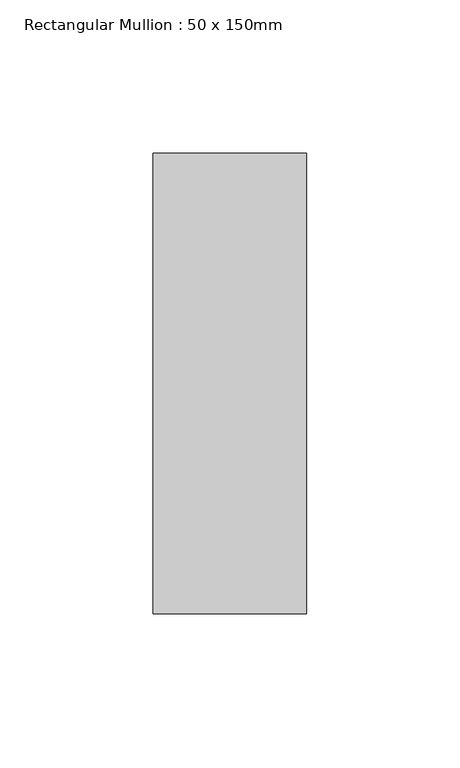
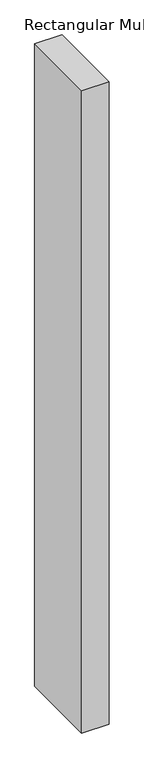
"""IFC4 building model written with IfcOpenShell, lengths in millimetres: member geometry, Rectangular Mullion : 50 x 150mm."""

import ifcopenshell
import ifcopenshell.guid

model = None  # the IFC model being written
_history = None  # IfcOwnerHistory: only IFC2X3 demands one
_inside = {}  # id of a spatial element -> (the spatial element, [elements in it])
_under = {}  # id of a project, library or spatial element -> (it, [spatial elements below it])
_declared = {}  # id of a project -> (the project, [libraries it declares])
_typed = {}  # id of a type object -> (the type object, [elements of that type])
_made_of = {}  # id of a material, layer set ... -> (it, [elements and type objects made of it])


def new_model(schema):
    """Start an empty IFC model of exactly this schema.

    Asked for "IFC4X3", IfcOpenShell would pick the latest addendum, in which some entities
    have other attributes; the version numbers below select the first issue.
    IFC2X3 requires an IfcOwnerHistory on every rooted entity: one is made here for all.
    """
    global model, _history
    if schema == "IFC4X3":
        model = ifcopenshell.file(schema_version=(4, 3, 0, 0))
    else:
        model = ifcopenshell.file(schema=schema)
    _inside.clear()
    _under.clear()
    _declared.clear()
    _typed.clear()
    _made_of.clear()
    _history = None
    if model.schema == "IFC2X3":
        org = make("IfcOrganization", Name="unknown")
        user = make(
            "IfcPersonAndOrganization",
            ThePerson=make("IfcPerson", FamilyName="unknown"),
            TheOrganization=org,
        )
        app = make(
            "IfcApplication",
            ApplicationDeveloper=org,
            Version="unknown",
            ApplicationFullName="unknown",
            ApplicationIdentifier="unknown",
        )
        _history = make(
            "IfcOwnerHistory",
            OwningUser=user,
            OwningApplication=app,
            ChangeAction="ADDED",
            CreationDate=0,
        )
    return model


def make(cls, **values):
    """One entity of the class cls with the attributes given. An attribute that is None is left unset."""
    return model.create_entity(
        cls, **{name: value for name, value in values.items() if value is not None}
    )


def rooted(cls, **values):
    """An entity with a GlobalId (a new one), such as an element, a storey or a relation."""
    return make(cls, GlobalId=ifcopenshell.guid.new(), OwnerHistory=_history, **values)


def si_unit(unit_type, name, prefix=None):
    """IfcSIUnit, for example si_unit("LENGTHUNIT", "METRE", prefix="MILLI")."""
    return make("IfcSIUnit", UnitType=unit_type, Prefix=prefix, Name=name)


def assignment(units):
    """IfcUnitAssignment: the units of a project."""
    return None if units is None else make("IfcUnitAssignment", Units=units)


def point(xyz):
    """IfcCartesianPoint."""
    return None if xyz is None else make("IfcCartesianPoint", Coordinates=xyz)


def direction(xyz):
    """IfcDirection."""
    return None if xyz is None else make("IfcDirection", DirectionRatios=xyz)


def frame(location, z_axis=None, x_axis=None):
    """IfcAxis2Placement3D, a coordinate frame: its origin and axes. An axis left out is left unset."""
    return make(
        "IfcAxis2Placement3D",
        Location=point(location),
        Axis=direction(z_axis),
        RefDirection=direction(x_axis),
    )


def origin():
    """The frame at (0, 0, 0) with its axes left unset."""
    return frame((0.0, 0.0, 0.0))


def place(relative_to, where):
    """IfcLocalPlacement: puts the frame where relative to a parent placement (None: the world)."""
    return make(
        "IfcLocalPlacement", PlacementRelTo=relative_to, RelativePlacement=where
    )


def context(
    kind, dimensions, precision=None, world=None, true_north=None, identifier=None
):
    """IfcGeometricRepresentationContext, for example the 3D "Model" context."""
    return make(
        "IfcGeometricRepresentationContext",
        ContextIdentifier=identifier,
        ContextType=kind,
        CoordinateSpaceDimension=dimensions,
        Precision=precision,
        WorldCoordinateSystem=world,
        TrueNorth=true_north,
    )


def project(units=None, contexts=None):
    """IfcProject with its units and contexts."""
    return rooted(
        "IfcProject",
        Name="project",
        RepresentationContexts=contexts,
        UnitsInContext=assignment(units),
    )


def spatial(cls, under=None, at=None, **own):
    """A site, building, storey or space (cls), placed at a placement, below another one or the project."""
    s = rooted(cls, ObjectPlacement=at, **own)
    if under is not None:
        _under.setdefault(under.id(), (under, []))[1].append(s)
    return s


def polyline(points):
    """IfcPolyline through the points."""
    return make("IfcPolyline", Points=[point(p) for p in points])


def outline(outer, holes=None, kind="AREA"):
    """IfcArbitraryClosedProfileDef: a profile drawn as a closed curve; with holes, ...WithVoids."""
    if holes is None:
        return make("IfcArbitraryClosedProfileDef", ProfileType=kind, OuterCurve=outer)
    return make(
        "IfcArbitraryProfileDefWithVoids",
        ProfileType=kind,
        OuterCurve=outer,
        InnerCurves=holes,
    )


def extrude(swept, where, along, depth):
    """IfcExtrudedAreaSolid: the profile swept, set in the frame where, extruded along a direction by depth."""
    return make(
        "IfcExtrudedAreaSolid",
        SweptArea=swept,
        Position=where,
        ExtrudedDirection=direction(along),
        Depth=depth,
    )


def shape(context_of_items, identifier, shape_type, items):
    """IfcShapeRepresentation: the items that make up one representation, for example the "Body"."""
    return make(
        "IfcShapeRepresentation",
        ContextOfItems=context_of_items,
        RepresentationIdentifier=identifier,
        RepresentationType=shape_type,
        Items=items,
    )


def source(mapping_origin, context_of_items, identifier, shape_type, items):
    """IfcRepresentationMap: a shape defined once, which mapped items show again and again."""
    return make(
        "IfcRepresentationMap",
        MappingOrigin=mapping_origin,
        MappedRepresentation=shape(context_of_items, identifier, shape_type, items),
    )


def transform(
    local_origin,
    x_axis=None,
    y_axis=None,
    z_axis=None,
    scale=None,
    scale2=None,
    scale3=None,
    uniform=True,
):
    """IfcCartesianTransformationOperator3D, or its non-uniform kind. x_axis, y_axis, z_axis: its Axis1, 2, 3."""
    if uniform:
        return make(
            "IfcCartesianTransformationOperator3D",
            Axis1=direction(x_axis),
            Axis2=direction(y_axis),
            LocalOrigin=point(local_origin),
            Scale=scale,
            Axis3=direction(z_axis),
        )
    return make(
        "IfcCartesianTransformationOperator3DnonUniform",
        Axis1=direction(x_axis),
        Axis2=direction(y_axis),
        LocalOrigin=point(local_origin),
        Scale=scale,
        Axis3=direction(z_axis),
        Scale2=scale2,
        Scale3=scale3,
    )


def mapped(mapping_source, mapping_target):
    """IfcMappedItem: shows the shape of a source again, moved by a transform."""
    return make(
        "IfcMappedItem", MappingSource=mapping_source, MappingTarget=mapping_target
    )


def made_of(thing, what):
    """Note that an element or type object is made of a material, layer set ...; save() writes the relation."""
    if what is not None:
        _made_of.setdefault(what.id(), (what, []))[1].append(thing)
    return thing


def element(
    cls,
    number,
    at=None,
    inside=None,
    cuts=None,
    type_object=None,
    material=None,
    context=None,
    identifier="Body",
    shape_type=None,
    held_by="IfcProductDefinitionShape",
    body=None,
    shapes=None,
    **own,
):
    """One element of the class cls, such as IfcWall. Its Tag is "e" and its number.

    at: its placement. inside: the storey or other place that contains it. cuts: it is an
    opening in that element (IfcRelVoidsElement). A single representation is given by context,
    identifier, shape_type and body (its items); several are given by shapes. held_by: the class
    of the entity that holds the representations. save() writes the other relations.
    """
    e = rooted(cls, Tag="e%d" % number, ObjectPlacement=at, **own)
    if body is not None:
        shapes = [shape(context, identifier, shape_type, body)]
    if shapes is not None:
        e.Representation = make(held_by, Representations=shapes)
    if inside is not None:
        _inside.setdefault(inside.id(), (inside, []))[1].append(e)
    if cuts is not None:
        rooted(
            "IfcRelVoidsElement", RelatingBuildingElement=cuts, RelatedOpeningElement=e
        )
    if type_object is not None:
        _typed.setdefault(type_object.id(), (type_object, []))[1].append(e)
    return made_of(e, material)


def aggregate(whole, parts):
    """IfcRelAggregates: a whole, such as a stair, and the parts it consists of."""
    return rooted("IfcRelAggregates", RelatingObject=whole, RelatedObjects=parts)


def save(model, path):
    """Write the relations noted so far, then the file.

    IfcRelAggregates (storeys below a building ...), IfcRelContainedInSpatialStructure (elements
    in a storey), IfcRelDefinesByType, IfcRelAssociatesMaterial and IfcRelDeclares: one each for
    every whole, place, type object, material and project.
    """
    for whole, parts in _under.values():
        aggregate(whole, parts)
    for where, things in _inside.values():
        rooted(
            "IfcRelContainedInSpatialStructure",
            RelatedElements=things,
            RelatingStructure=where,
        )
    for kind, things in _typed.values():
        rooted("IfcRelDefinesByType", RelatedObjects=things, RelatingType=kind)
    for what, things in _made_of.values():
        rooted("IfcRelAssociatesMaterial", RelatedObjects=things, RelatingMaterial=what)
    for by, libraries in _declared.values():
        rooted("IfcRelDeclares", RelatingContext=by, RelatedDefinitions=libraries)
    model.write(path)


def rectangular_mullion_50_x_150mm_8d7ec0e8(model_context):
    return source(origin(), model_context, "Body", "SweptSolid", [
        extrude(outline(polyline([(0.0, 75.0), (0.0, -75.0), (-50.0, -75.0), (-50.0, 75.0), (0.0, 75.0)])), frame((0.0, 0.0, -1250.0000002), z_axis=(0.0, 0.0, 1.0), x_axis=(1.0, 0.0, 0.0)), (0.0, 0.0, 1.0), 1250.0000002),
    ])


if __name__ == "__main__":
    model = new_model("IFC4")
    model_context = context("Model", 3, world=origin())
    ifc_project = project(units=[si_unit("LENGTHUNIT", "METRE", prefix="MILLI")], contexts=[model_context])
    site = spatial("IfcSite", under=ifc_project)
    building = spatial("IfcBuilding", under=site)
    placement = place(None, origin())
    rectangular_mullion_50_x_150mm_shape = rectangular_mullion_50_x_150mm_8d7ec0e8(model_context)
    element("IfcMember", 1, ObjectType="Rectangular Mullion : 50 x 150mm", at=placement, inside=building, context=model_context, shape_type="MappedRepresentation", body=[
        mapped(rectangular_mullion_50_x_150mm_shape, transform((0.0, 0.0, 0.0), x_axis=(1.0, 0.0, 0.0), y_axis=(0.0, 1.0, 0.0), z_axis=(0.0, 0.0, 1.0))),
    ])
    save(model, "model.ifc")

# Revit data of these elements
# Type "Rectangular Mullion : 50 x 150mm"
#   built-in parameter 1007304 = 0.492126 (stored number, unit not read)
#   built-in parameter 1007301 = 0.082021 (stored number, unit not read)
#   built-in parameter 1007300 = 0.082021 (stored number, unit not read)
# Element 1 (IfcMember, "Rectangular Mullion : 50 x 150mm")
#   Materials on its faces: "Aluminium"
# Materials
#   "Aluminium": class "Metal", colour RGB 247 247 247, transparency 0, Description = "Aluminium 6061", Cost = 0
